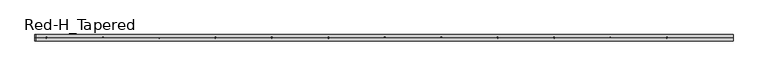
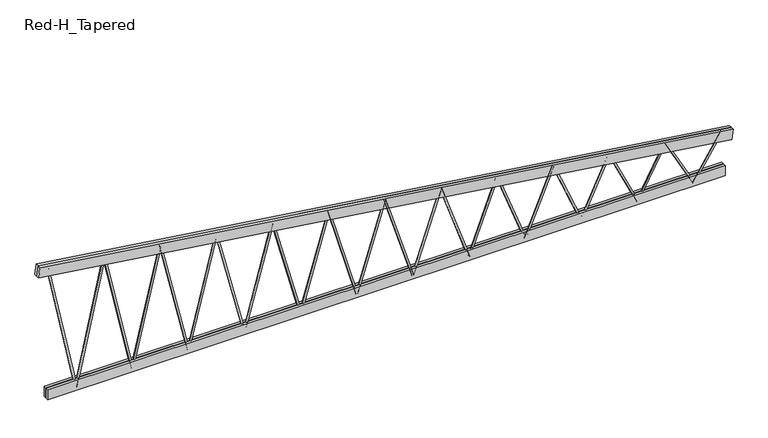
"""IFC4 building model written with IfcOpenShell, lengths in millimetres: beam geometry, Construction_Frames_RedBuilt_Openweb_Red-H_Tapered : Red-H_Tapered."""

from ifc_helpers import new_model, si_unit, point, frame, origin, origin_2d, place, context, project, spatial, polyline, circle_curve, trimmed, segment, composite_curve, outline, extrude, source, transform, mapped, element, save


def red_h_tapered_31e13fe1(model_context):
    return source(origin(), model_context, "Body", "SweptSolid", [
        extrude(outline(composite_curve([segment(trimmed(circle_curve(origin_2d(), 12.7), [point((0.0, -12.7))], [point((0.0, 12.7))], False, "CARTESIAN"), True, "CONTINUOUS"), segment(trimmed(circle_curve(origin_2d(), 12.7), [point((0.0, 12.7))], [point((0.0, -12.7))], False, "CARTESIAN"), True, "CONTINUOUS")], self_intersect=False)), frame((-368.763372, 0.0, -367.0101562), z_axis=(-0.27698303070668895, 0.0, 0.9608748101082354), x_axis=(0.0, -1.0, 0.0)), (0.0, 0.0, 1.0), 1331.3572714),
        extrude(outline(composite_curve([segment(trimmed(circle_curve(origin_2d(), 12.7), [point((0.0, 12.7))], [point((0.0, -12.7))], False, "CARTESIAN"), True, "CONTINUOUS"), segment(trimmed(circle_curve(origin_2d(), 12.7), [point((0.0, -12.7))], [point((0.0, 12.7))], False, "CARTESIAN"), True, "CONTINUOUS")], self_intersect=False)), frame((-1106.2901159, 0.0, -367.0101562), z_axis=(0.2769830307066903, 0.0, 0.9608748101082351), x_axis=(0.0, -1.0, 0.0)), (0.0, 0.0, 1.0), 1331.3572714),
        extrude(outline(composite_curve([segment(trimmed(circle_curve(origin_2d(), 12.7), [point((0.0, -12.7000001))], [point((0.0, 12.6999999))], False, "CARTESIAN"), True, "CONTINUOUS"), segment(trimmed(circle_curve(origin_2d(), 12.7), [point((0.0, 12.6999999))], [point((0.0, -12.7000001))], False, "CARTESIAN"), True, "CONTINUOUS")], self_intersect=False)), frame((-1106.2901159, 0.0, -367.0101562), z_axis=(-0.2584126885234393, 0.0, 0.9660346176044045), x_axis=(0.0, -1.0, 0.0)), (0.0, 0.0, 1.0), 1427.0327594),
        extrude(outline(composite_curve([segment(trimmed(circle_curve(origin_2d(), 12.7), [point((0.0, -12.6999999))], [point((0.0, 12.7000001))], False, "CARTESIAN"), True, "CONTINUOUS"), segment(trimmed(circle_curve(origin_2d(), 12.7), [point((0.0, 12.7000001))], [point((0.0, -12.6999999))], False, "CARTESIAN"), True, "CONTINUOUS")], self_intersect=False)), frame((-1843.8168599, 0.0, -367.0101562), z_axis=(0.25841268852344296, 0.0, 0.9660346176044036), x_axis=(0.0, -1.0, 0.0)), (0.0, 0.0, 1.0), 1427.0327594),
        extrude(outline(composite_curve([segment(trimmed(circle_curve(origin_2d(), 12.7), [point((0.0, 12.7))], [point((0.0, -12.7))], False, "CARTESIAN"), True, "CONTINUOUS"), segment(trimmed(circle_curve(origin_2d(), 12.7), [point((0.0, -12.7))], [point((0.0, 12.7))], False, "CARTESIAN"), True, "CONTINUOUS")], self_intersect=False)), frame((-1843.8168599, 0.0, -367.0101562), z_axis=(-0.24210230390417398, 0.0, 0.9702507276185321), x_axis=(0.0, -1.0, 0.0)), (0.0, 0.0, 1.0), 1523.1716759),
        extrude(outline(composite_curve([segment(trimmed(circle_curve(origin_2d(), 12.7), [point((0.0, -12.7))], [point((0.0, 12.7))], False, "CARTESIAN"), True, "CONTINUOUS"), segment(trimmed(circle_curve(origin_2d(), 12.7), [point((0.0, 12.7))], [point((0.0, -12.7))], False, "CARTESIAN"), True, "CONTINUOUS")], self_intersect=False)), frame((-2581.3436038, 0.0, -367.0101562), z_axis=(0.24210230390417306, 0.0, 0.9702507276185324), x_axis=(0.0, -1.0, 0.0)), (0.0, 0.0, 1.0), 1523.1716759),
        extrude(outline(composite_curve([segment(trimmed(circle_curve(origin_2d(), 12.7), [point((0.0, 12.6999999))], [point((0.0, -12.7))], False, "CARTESIAN"), True, "CONTINUOUS"), segment(trimmed(circle_curve(origin_2d(), 12.7), [point((0.0, -12.7))], [point((0.0, 12.6999999))], False, "CARTESIAN"), True, "CONTINUOUS")], self_intersect=False)), frame((-2581.3436038, 0.0, -367.0101562), z_axis=(-0.22767506764539427, 0.0, 0.9737371634957069), x_axis=(0.0, -1.0, 0.0)), (0.0, 0.0, 1.0), 1619.6915007),
        extrude(outline(composite_curve([segment(trimmed(circle_curve(origin_2d(), 12.7), [point((0.0, -12.7))], [point((0.0, 12.7))], False, "CARTESIAN"), True, "CONTINUOUS"), segment(trimmed(circle_curve(origin_2d(), 12.7), [point((0.0, 12.7))], [point((0.0, -12.7))], False, "CARTESIAN"), True, "CONTINUOUS")], self_intersect=False)), frame((-3318.8703478, 0.0, -367.0101562), z_axis=(0.227675067645399, 0.0, 0.9737371634957059), x_axis=(0.0, -1.0, 0.0)), (0.0, 0.0, 1.0), 1619.6915007),
        extrude(outline(composite_curve([segment(trimmed(circle_curve(origin_2d(), 12.7), [point((0.0, 12.7))], [point((0.0, -12.7))], False, "CARTESIAN"), True, "CONTINUOUS"), segment(trimmed(circle_curve(origin_2d(), 12.7), [point((0.0, -12.7))], [point((0.0, 12.7))], False, "CARTESIAN"), True, "CONTINUOUS")], self_intersect=False)), frame((-3318.8703478, 0.0, -367.0101562), z_axis=(-0.2148309706016159, 0.0, 0.9766512448516961), x_axis=(0.0, -1.0, 0.0)), (0.0, 0.0, 1.0), 1716.5279799),
        extrude(outline(composite_curve([segment(trimmed(circle_curve(origin_2d(), 12.7), [point((0.0, -12.7000001))], [point((0.0, 12.7))], False, "CARTESIAN"), True, "CONTINUOUS"), segment(trimmed(circle_curve(origin_2d(), 12.7), [point((0.0, 12.7))], [point((0.0, -12.7000001))], False, "CARTESIAN"), True, "CONTINUOUS")], self_intersect=False)), frame((-4056.3970917, 0.0, -367.0101562), z_axis=(0.21483097060161488, 0.0, 0.9766512448516963), x_axis=(0.0, -1.0, 0.0)), (0.0, 0.0, 1.0), 1716.5279799),
        extrude(outline(composite_curve([segment(trimmed(circle_curve(origin_2d(), 12.7), [point((0.0, 12.7))], [point((0.0, -12.7000001))], False, "CARTESIAN"), True, "CONTINUOUS"), segment(trimmed(circle_curve(origin_2d(), 12.7), [point((0.0, -12.7000001))], [point((0.0, 12.7))], False, "CARTESIAN"), True, "CONTINUOUS")], self_intersect=False)), frame((-4056.3970917, 0.0, -367.0101562), z_axis=(-0.20332884449837235, 0.0, 0.9791105049967327), x_axis=(0.0, -1.0, 0.0)), (0.0, 0.0, 1.0), 1813.6303921),
        extrude(outline(composite_curve([segment(trimmed(circle_curve(origin_2d(), 12.7), [point((0.0, 12.7))], [point((0.0, -12.6999999))], False, "CARTESIAN"), True, "CONTINUOUS"), segment(trimmed(circle_curve(origin_2d(), 12.7), [point((0.0, -12.6999999))], [point((0.0, 12.7))], False, "CARTESIAN"), True, "CONTINUOUS")], self_intersect=False)), frame((4056.3970917, 0.0, -367.0101562), z_axis=(0.5337808022114843, 0.0, 0.8456228800064863), x_axis=(0.0, -1.0, 0.0)), (0.0, 0.0, 1.0), 690.851695),
        extrude(outline(composite_curve([segment(trimmed(circle_curve(origin_2d(), 12.7), [point((0.0, -12.7))], [point((0.0, 12.7))], False, "CARTESIAN"), True, "CONTINUOUS"), segment(trimmed(circle_curve(origin_2d(), 12.7), [point((0.0, 12.7))], [point((0.0, -12.7))], False, "CARTESIAN"), True, "CONTINUOUS")], self_intersect=False)), frame((4056.3970917, 0.0, -367.0101562), z_axis=(-0.4748257487781058, 0.0, 0.8800798306388525), x_axis=(0.0, -1.0, 0.0)), (0.0, 0.0, 1.0), 776.6288432),
        extrude(outline(composite_curve([segment(trimmed(circle_curve(origin_2d(), 12.7), [point((0.0, 12.7))], [point((0.0, -12.7))], False, "CARTESIAN"), True, "CONTINUOUS"), segment(trimmed(circle_curve(origin_2d(), 12.7), [point((0.0, -12.7))], [point((0.0, 12.7))], False, "CARTESIAN"), True, "CONTINUOUS")], self_intersect=False)), frame((3318.8703478, 0.0, -367.0101562), z_axis=(0.4748257487781032, 0.0, 0.8800798306388539), x_axis=(0.0, -1.0, 0.0)), (0.0, 0.0, 1.0), 776.6288432),
        extrude(outline(composite_curve([segment(trimmed(circle_curve(origin_2d(), 12.7), [point((0.0, -12.7))], [point((0.0, 12.7))], False, "CARTESIAN"), True, "CONTINUOUS"), segment(trimmed(circle_curve(origin_2d(), 12.7), [point((0.0, 12.7))], [point((0.0, -12.7))], False, "CARTESIAN"), True, "CONTINUOUS")], self_intersect=False)), frame((3318.8703478, 0.0, -367.0101562), z_axis=(-0.4261671768998602, 0.0, 0.904644425911752), x_axis=(0.0, -1.0, 0.0)), (0.0, 0.0, 1.0), 865.3021442),
        extrude(outline(composite_curve([segment(trimmed(circle_curve(origin_2d(), 12.7), [point((0.0, 12.7))], [point((0.0, -12.7))], False, "CARTESIAN"), True, "CONTINUOUS"), segment(trimmed(circle_curve(origin_2d(), 12.7), [point((0.0, -12.7))], [point((0.0, 12.7))], False, "CARTESIAN"), True, "CONTINUOUS")], self_intersect=False)), frame((2581.3436038, 0.0, -367.0101562), z_axis=(0.42616717689985956, 0.0, 0.9046444259117523), x_axis=(0.0, -1.0, 0.0)), (0.0, 0.0, 1.0), 865.3021442),
        extrude(outline(composite_curve([segment(trimmed(circle_curve(origin_2d(), 12.7), [point((0.0, -12.7))], [point((0.0, 12.7))], False, "CARTESIAN"), True, "CONTINUOUS"), segment(trimmed(circle_curve(origin_2d(), 12.7), [point((0.0, 12.7))], [point((0.0, -12.7))], False, "CARTESIAN"), True, "CONTINUOUS")], self_intersect=False)), frame((2581.3436038, 0.0, -367.0101562), z_axis=(-0.385709076088184, 0.0, 0.9226204575139224), x_axis=(0.0, -1.0, 0.0)), (0.0, 0.0, 1.0), 956.0660997),
        extrude(outline(composite_curve([segment(trimmed(circle_curve(origin_2d(), 12.7), [point((0.0, 12.7))], [point((0.0, -12.7))], False, "CARTESIAN"), True, "CONTINUOUS"), segment(trimmed(circle_curve(origin_2d(), 12.7), [point((0.0, -12.7))], [point((0.0, 12.7))], False, "CARTESIAN"), True, "CONTINUOUS")], self_intersect=False)), frame((1843.8168599, 0.0, -367.0101562), z_axis=(0.3857090760881839, 0.0, 0.9226204575139225), x_axis=(0.0, -1.0, 0.0)), (0.0, 0.0, 1.0), 956.0660997),
        extrude(outline(composite_curve([segment(trimmed(circle_curve(origin_2d(), 12.7), [point((0.0, -12.7))], [point((0.0, 12.7))], False, "CARTESIAN"), True, "CONTINUOUS"), segment(trimmed(circle_curve(origin_2d(), 12.7), [point((0.0, 12.7))], [point((0.0, -12.7))], False, "CARTESIAN"), True, "CONTINUOUS")], self_intersect=False)), frame((1843.8168599, 0.0, -367.0101562), z_axis=(-0.35174662614127256, 0.0, 0.9360952467554954), x_axis=(0.0, -1.0, 0.0)), (0.0, 0.0, 1.0), 1048.3778509),
        extrude(outline(composite_curve([segment(trimmed(circle_curve(origin_2d(), 12.7), [point((0.0, 12.7000001))], [point((0.0, -12.7))], False, "CARTESIAN"), True, "CONTINUOUS"), segment(trimmed(circle_curve(origin_2d(), 12.7), [point((0.0, -12.7))], [point((0.0, 12.7000001))], False, "CARTESIAN"), True, "CONTINUOUS")], self_intersect=False)), frame((1106.2901159, 0.0, -367.0101562), z_axis=(0.3517466261412766, 0.0, 0.9360952467554939), x_axis=(0.0, -1.0, 0.0)), (0.0, 0.0, 1.0), 1048.3778509),
        extrude(outline(composite_curve([segment(trimmed(circle_curve(origin_2d(), 12.7), [point((0.0, -12.7))], [point((0.0, 12.7))], False, "CARTESIAN"), True, "CONTINUOUS"), segment(trimmed(circle_curve(origin_2d(), 12.7), [point((0.0, 12.7))], [point((0.0, -12.7))], False, "CARTESIAN"), True, "CONTINUOUS")], self_intersect=False)), frame((1106.2901159, 0.0, -367.0101562), z_axis=(-0.32294913767070077, 0.0, 0.9464163219628827), x_axis=(0.0, -1.0, 0.0)), (0.0, 0.0, 1.0), 1141.8620735),
        extrude(outline(composite_curve([segment(trimmed(circle_curve(origin_2d(), 12.7), [point((0.0, 12.7))], [point((0.0, -12.7))], False, "CARTESIAN"), True, "CONTINUOUS"), segment(trimmed(circle_curve(origin_2d(), 12.7), [point((0.0, -12.7))], [point((0.0, 12.7))], False, "CARTESIAN"), True, "CONTINUOUS")], self_intersect=False)), frame((368.763372, 0.0, -367.0101562), z_axis=(0.32294913767070255, 0.0, 0.9464163219628822), x_axis=(0.0, -1.0, 0.0)), (0.0, 0.0, 1.0), 1141.8620735),
        extrude(outline(composite_curve([segment(trimmed(circle_curve(origin_2d(), 12.7), [point((0.0, -12.7))], [point((0.0, 12.7))], False, "CARTESIAN"), True, "CONTINUOUS"), segment(trimmed(circle_curve(origin_2d(), 12.7), [point((0.0, 12.7))], [point((0.0, -12.7))], False, "CARTESIAN"), True, "CONTINUOUS")], self_intersect=False)), frame((368.763372, 0.0, -367.0101562), z_axis=(-0.2982912299156644, 0.0, 0.9544749038897777), x_axis=(0.0, -1.0, 0.0)), (0.0, 0.0, 1.0), 1236.2528127),
        extrude(outline(composite_curve([segment(trimmed(circle_curve(origin_2d(), 12.7), [point((0.0, 12.7))], [point((0.0, -12.7))], False, "CARTESIAN"), True, "CONTINUOUS"), segment(trimmed(circle_curve(origin_2d(), 12.7), [point((0.0, -12.7))], [point((0.0, 12.7))], False, "CARTESIAN"), True, "CONTINUOUS")], self_intersect=False)), frame((-368.763372, 0.0, -367.0101562), z_axis=(0.29829122991562734, 0.0, 0.9544749038897892), x_axis=(0.0, -1.0, 0.0)), (0.0, 0.0, 1.0), 1236.2528127),
        extrude(outline(polyline([(-4450.5604637, -41.275), (-4450.5604637, -3.175), (4450.5604637, -3.175), (4450.5604637, -41.275), (-4450.5604637, -41.275)])), frame((0.0, 0.0, -386.0601562), z_axis=(0.0, 0.0, 1.0), x_axis=(1.0, 0.0, 0.0)), (0.0, 0.0, 1.0), 139.7),
        extrude(outline(polyline([(-4450.5604637, 3.175), (-4450.5604637, 41.275), (4450.5604637, 41.275), (4450.5604637, 3.175), (-4450.5604637, 3.175)])), frame((0.0, 0.0, -386.0601562), z_axis=(0.0, 0.0, 1.0), x_axis=(1.0, 0.0, 0.0)), (0.0, 0.0, 1.0), 139.7),
        extrude(outline(polyline([(0.0, -38.1), (0.0, 0.0), (9191.3797279, 0.0), (9191.3797279, -38.1), (0.0, -38.1)])), frame((-4571.3425818, -3.175, 1347.2255525), z_axis=(0.13730936348531744, 0.0, 0.9905282119653418), x_axis=(0.9905282119653418, 0.0, -0.13730936348531744)), (0.0, 0.0, 1.0), 139.7),
        extrude(outline(polyline([(0.0, -38.1), (0.0, 0.0), (9191.3797279, 0.0), (9191.3797279, -38.1), (0.0, -38.1)])), frame((-4571.3425818, 41.275, 1347.2255525), z_axis=(0.13730936348531744, 0.0, 0.9905282119653418), x_axis=(0.9905282119653418, 0.0, -0.13730936348531744)), (0.0, 0.0, 1.0), 139.7),
    ])


if __name__ == "__main__":
    model = new_model("IFC4")
    model_context = context("Model", 3, world=origin())
    ifc_project = project(units=[si_unit("LENGTHUNIT", "METRE", prefix="MILLI")], contexts=[model_context])
    site = spatial("IfcSite", under=ifc_project)
    building = spatial("IfcBuilding", under=site)
    placement = place(None, origin())
    red_h_tapered_shape = red_h_tapered_31e13fe1(model_context)
    element("IfcBeam", 1, ObjectType="Construction_Frames_RedBuilt_Openweb_Red-H_Tapered : Red-H_Tapered", at=placement, inside=building, context=model_context, shape_type="MappedRepresentation", body=[
        mapped(red_h_tapered_shape, transform((0.0, 0.0, 0.0), x_axis=(1.0, 0.0, 0.0), y_axis=(0.0, 1.0, 0.0), z_axis=(0.0, 0.0, 1.0))),
    ])
    save(model, "model.ifc")

# Revit data of these elements
# Type "Construction_Frames_RedBuilt_Openweb_Red-H_Tapered : Red-H_Tapered"
#   Youtube clip = ""
#   Weight Net (Kg) = "0"
#   Webs = "Up to 2\" diameter tubular steel"
#   Uniformat II Description = ""
#   Uniformat II Code = ""
#   Uniclass 2015 Name = "Softwood trusses"
#   Uniclass 2015 Code = "Pr_20_85_90_81"
#   Uniclass 2.0 Description = "Structural Framing Systems"
#   Uniclass 2.0 Code = "SS-15-10-75"
#   Uniclass 1.4 Description = "Trusses"
#   Uniclass 1.4 Code = "L3523"
#   UNSPSC Code = "30103606"
#   Technical description = "http://www.redbuilt.com/reference/literature-and-other-resources"
#   Region South America = "None"
#   Region Oceania = "None"
#   Region North America = "US"
#   Region Middle East = "None"
#   Region Europe = "None"
#   Region Asia = "None"
#   Region Antarctica = "None"
#   Region Africa = "None"
#   QR code = "http://bimobject.com/redbuilt/product/redbuilt-0003"
#   Product url = "http://www.redbuilt.com/products/default.aspx?id=2"
#   Product group = "Wood Trusses"
#   Product family = "Construction"
#   Product data url = "https://bimobject.com/redbuilt/product/redbuilt-0003"
#   Product certification = ""
#   Product SKU = "redbuilt-0003"
#   Product Page URL = "http://www.redbuilt.com/commercial-systems/red-m-red-h-open-web-trusses"
#   Product Guid = "2c5793f2-6ffb-4665-b825-cf90c048e711"
#   Product Documentation Link = "http://www.redbuilt.com/documents/OW_Guide_2017_07_LowRes_wLinks.pdf"
#   OmniClass Description = "Wood Trusses"
#   OmniClass Code = "23-13 35 19 13 17"
#   NBS Reference Description = ""
#   NBS Reference Code = ""
#   Material secondary = "Steel"
#   Material main = "Wood"
#   Masterformat 2014 Description = "Metal-Web Wood Joists"
#   Masterformat 2014 Code = "06 17 36"
#   Manufacturer name = "RedBuilt"
#   Manufacturer country = "United States"
#   Installation instructions = "http://www.redbuilt.com/documents/Installation_Sheets_Open-Web.pdf"
#   IFC Classification = ""
#   EAN code = ""
#   Design country = "United States"
#   Product Information = "http://redbuilt.com/products/default.aspx?id=2"
#   Model = "Red-H-Tapered"
#   Manufacturer URL = "http://redbuilt.com/"
#   Manufacturer = "RedBuilt™"
#   Description = "Open Web Truss"
#   Date of publishing = "8/17/2010"
#   Contact us = "http://redbuilt.com/contact/"
#   Chords = "Double 1½\" x 5½\" MSR lumber"
#   COBIe Type Category = ""
#   Brand url = "http://www.redbuilt.com"
#   BIMobject main category code = "construction"
#   BIMobject main category = "Construction"
#   BIMobject category code = "construction-frames-trusses"
#   BIMobject category = "Frames & Trusses"
#   Web Radius = 0' - 0 1/2"
#   Web Layout Offset Start [instance default] = 0' - 5"
#   Web Layout Offset End [instance default] = 0' - 5"
#   Web Diameter = 0' - 1"
#   TotalLength [instance default] = 20' - 0"
#   Span Minimum = 4' - 0"
#   Span Maximum = 70' - 0"
#   Span Limit [instance default] = 20' - 0"
#   Nominal width = 0' - 0"
#   Nominal height = 0' - 0"
#   Inner Depth Top [instance default] = 0' - 2.76372"
#   Depth Start [instance default] = 6' - 0"
#   Top Chord Length [instance default] = 20' - 1.19701"
#   TC Extension Start Aux [instance default] = 0' - 0"
#   TC Extension End Aux [instance default] = 0' - 0"
#   T-B Chord Length Difference L [instance default] = 0' - 4"
#   T-B Chord Length Difference [instance default] = 0' - 4"
#   Height 2 [instance default] = 6' - 0"
#   Depth Minimum at Wall = 2' - 0"
#   Depth Maximum at Wall = 6' - 0"
#   Depth Lower End [instance default] = 2' - 0"
#   Depth Higher End [instance default] = 6' - 0"
#   Depth End [instance default] = 2' - 0"
#   Depth 2 [instance default] = 2' - 0"
#   Chord Width = 0' - 3 1/4"
#   Chord Thickness = 0' - 1 1/2"
#   Chord Depth = 0' - 5 1/2"
#   Offset Start [instance default] = 0' - 0"
#   TC Extension Start [instance default] = 0' - 0"
#   End Panel = 0' - 5"
#   Offset End [instance default] = 0' - 0"
#   TC Extension End [instance default] = 0' - 0"
#   Length [instance default] = 20' - 0"
#   Angle [instance default] = 5.71059°
#   Span Limit Warning [instance default] = no
#   Edition number = 1
#   Top Bearing Start [instance default] = yes
#   Top Bearing End [instance default] = yes
#   Bottom Bearing Start [instance default] = no
#   Bottom Bearing End [instance default] = no
#   8 Panels [instance default] = yes
#   16 Panels [instance default] = no
#   12 Panels [instance default] = no
#   Web Material = RedBuilt-Steel, Galvanized
#   Clip Material = RedBuilt-Steel, Galvanized
#   Chords Material = RedBuilt-MSR
#   URL = ""
#   Assembly Code = ""
# Element 1 (IfcBeam, "Construction_Frames_RedBuilt_Openweb_Red-H_Tapered : Red-H_Tapered")
#   TotalLength = 29' - 10.43783"
#   Span Limit = 29' - 10.43783"
#   Inner Depth Top = 0' - 2.7763"
#   Top Chord Length = 30' - 1.86534"
#   Depth 2 = 4' - 1 11/16"
#   Angle = 7.89218°
#   8 Panels = no
#   12 Panels = yes
#   Materials on its faces: "RedBuilt-Steel, Galvanized", "RedBuilt-MSR"
# Materials
#   "RedBuilt-Steel, Galvanized": class "Metal", colour RGB 164 172 176, transparency 0, Manufacturer = "RedBuilt. LLC", Comments = "Openweb Metal Web", URL = "http://www.redbuilt.com/", Description = "Galvanized steel", Cost = 0
#   "RedBuilt-MSR": class "Wood", colour RGB 213 182 136, transparency 0, Manufacturer = "RedBuilt, LLC", URL = "http://www.redbuilt.com/", Cost = 0
